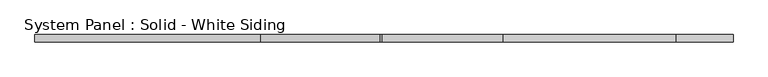
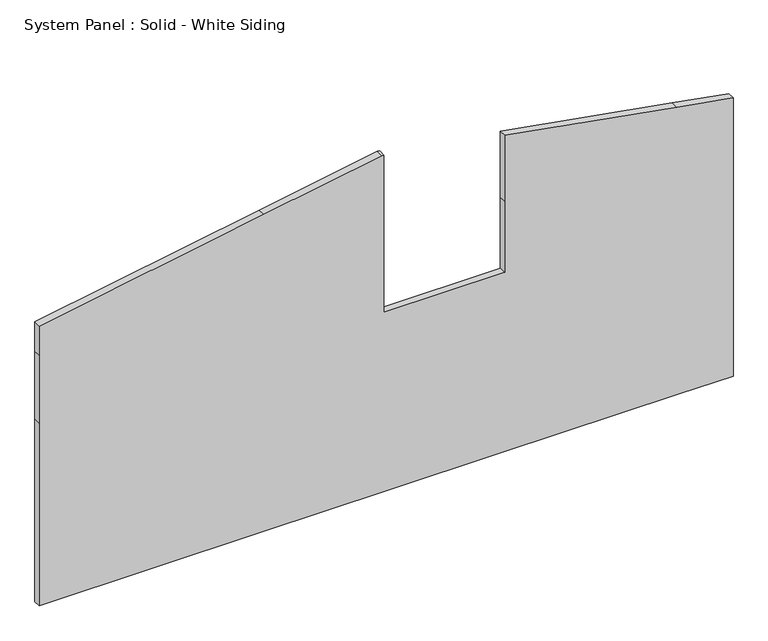
"""IFC4 building model written with IfcOpenShell, lengths in millimetres: plate geometry, System Panel : Solid - White Siding."""

import ifcopenshell
import ifcopenshell.guid

model = None  # the IFC model being written
_history = None  # IfcOwnerHistory: only IFC2X3 demands one
_inside = {}  # id of a spatial element -> (the spatial element, [elements in it])
_under = {}  # id of a project, library or spatial element -> (it, [spatial elements below it])
_declared = {}  # id of a project -> (the project, [libraries it declares])
_typed = {}  # id of a type object -> (the type object, [elements of that type])
_made_of = {}  # id of a material, layer set ... -> (it, [elements and type objects made of it])


def new_model(schema):
    """Start an empty IFC model of exactly this schema.

    Asked for "IFC4X3", IfcOpenShell would pick the latest addendum, in which some entities
    have other attributes; the version numbers below select the first issue.
    IFC2X3 requires an IfcOwnerHistory on every rooted entity: one is made here for all.
    """
    global model, _history
    if schema == "IFC4X3":
        model = ifcopenshell.file(schema_version=(4, 3, 0, 0))
    else:
        model = ifcopenshell.file(schema=schema)
    _inside.clear()
    _under.clear()
    _declared.clear()
    _typed.clear()
    _made_of.clear()
    _history = None
    if model.schema == "IFC2X3":
        org = make("IfcOrganization", Name="unknown")
        user = make(
            "IfcPersonAndOrganization",
            ThePerson=make("IfcPerson", FamilyName="unknown"),
            TheOrganization=org,
        )
        app = make(
            "IfcApplication",
            ApplicationDeveloper=org,
            Version="unknown",
            ApplicationFullName="unknown",
            ApplicationIdentifier="unknown",
        )
        _history = make(
            "IfcOwnerHistory",
            OwningUser=user,
            OwningApplication=app,
            ChangeAction="ADDED",
            CreationDate=0,
        )
    return model


def make(cls, **values):
    """One entity of the class cls with the attributes given. An attribute that is None is left unset."""
    return model.create_entity(
        cls, **{name: value for name, value in values.items() if value is not None}
    )


def rooted(cls, **values):
    """An entity with a GlobalId (a new one), such as an element, a storey or a relation."""
    return make(cls, GlobalId=ifcopenshell.guid.new(), OwnerHistory=_history, **values)


def si_unit(unit_type, name, prefix=None):
    """IfcSIUnit, for example si_unit("LENGTHUNIT", "METRE", prefix="MILLI")."""
    return make("IfcSIUnit", UnitType=unit_type, Prefix=prefix, Name=name)


def assignment(units):
    """IfcUnitAssignment: the units of a project."""
    return None if units is None else make("IfcUnitAssignment", Units=units)


def point(xyz):
    """IfcCartesianPoint."""
    return None if xyz is None else make("IfcCartesianPoint", Coordinates=xyz)


def direction(xyz):
    """IfcDirection."""
    return None if xyz is None else make("IfcDirection", DirectionRatios=xyz)


def frame(location, z_axis=None, x_axis=None):
    """IfcAxis2Placement3D, a coordinate frame: its origin and axes. An axis left out is left unset."""
    return make(
        "IfcAxis2Placement3D",
        Location=point(location),
        Axis=direction(z_axis),
        RefDirection=direction(x_axis),
    )


def origin():
    """The frame at (0, 0, 0) with its axes left unset."""
    return frame((0.0, 0.0, 0.0))


def place(relative_to, where):
    """IfcLocalPlacement: puts the frame where relative to a parent placement (None: the world)."""
    return make(
        "IfcLocalPlacement", PlacementRelTo=relative_to, RelativePlacement=where
    )


def context(
    kind, dimensions, precision=None, world=None, true_north=None, identifier=None
):
    """IfcGeometricRepresentationContext, for example the 3D "Model" context."""
    return make(
        "IfcGeometricRepresentationContext",
        ContextIdentifier=identifier,
        ContextType=kind,
        CoordinateSpaceDimension=dimensions,
        Precision=precision,
        WorldCoordinateSystem=world,
        TrueNorth=true_north,
    )


def project(units=None, contexts=None):
    """IfcProject with its units and contexts."""
    return rooted(
        "IfcProject",
        Name="project",
        RepresentationContexts=contexts,
        UnitsInContext=assignment(units),
    )


def spatial(cls, under=None, at=None, **own):
    """A site, building, storey or space (cls), placed at a placement, below another one or the project."""
    s = rooted(cls, ObjectPlacement=at, **own)
    if under is not None:
        _under.setdefault(under.id(), (under, []))[1].append(s)
    return s


def polyline(points):
    """IfcPolyline through the points."""
    return make("IfcPolyline", Points=[point(p) for p in points])


def outline(outer, holes=None, kind="AREA"):
    """IfcArbitraryClosedProfileDef: a profile drawn as a closed curve; with holes, ...WithVoids."""
    if holes is None:
        return make("IfcArbitraryClosedProfileDef", ProfileType=kind, OuterCurve=outer)
    return make(
        "IfcArbitraryProfileDefWithVoids",
        ProfileType=kind,
        OuterCurve=outer,
        InnerCurves=holes,
    )


def extrude(swept, where, along, depth):
    """IfcExtrudedAreaSolid: the profile swept, set in the frame where, extruded along a direction by depth."""
    return make(
        "IfcExtrudedAreaSolid",
        SweptArea=swept,
        Position=where,
        ExtrudedDirection=direction(along),
        Depth=depth,
    )


def shape(context_of_items, identifier, shape_type, items):
    """IfcShapeRepresentation: the items that make up one representation, for example the "Body"."""
    return make(
        "IfcShapeRepresentation",
        ContextOfItems=context_of_items,
        RepresentationIdentifier=identifier,
        RepresentationType=shape_type,
        Items=items,
    )


def source(mapping_origin, context_of_items, identifier, shape_type, items):
    """IfcRepresentationMap: a shape defined once, which mapped items show again and again."""
    return make(
        "IfcRepresentationMap",
        MappingOrigin=mapping_origin,
        MappedRepresentation=shape(context_of_items, identifier, shape_type, items),
    )


def transform(
    local_origin,
    x_axis=None,
    y_axis=None,
    z_axis=None,
    scale=None,
    scale2=None,
    scale3=None,
    uniform=True,
):
    """IfcCartesianTransformationOperator3D, or its non-uniform kind. x_axis, y_axis, z_axis: its Axis1, 2, 3."""
    if uniform:
        return make(
            "IfcCartesianTransformationOperator3D",
            Axis1=direction(x_axis),
            Axis2=direction(y_axis),
            LocalOrigin=point(local_origin),
            Scale=scale,
            Axis3=direction(z_axis),
        )
    return make(
        "IfcCartesianTransformationOperator3DnonUniform",
        Axis1=direction(x_axis),
        Axis2=direction(y_axis),
        LocalOrigin=point(local_origin),
        Scale=scale,
        Axis3=direction(z_axis),
        Scale2=scale2,
        Scale3=scale3,
    )


def mapped(mapping_source, mapping_target):
    """IfcMappedItem: shows the shape of a source again, moved by a transform."""
    return make(
        "IfcMappedItem", MappingSource=mapping_source, MappingTarget=mapping_target
    )


def made_of(thing, what):
    """Note that an element or type object is made of a material, layer set ...; save() writes the relation."""
    if what is not None:
        _made_of.setdefault(what.id(), (what, []))[1].append(thing)
    return thing


def element(
    cls,
    number,
    at=None,
    inside=None,
    cuts=None,
    type_object=None,
    material=None,
    context=None,
    identifier="Body",
    shape_type=None,
    held_by="IfcProductDefinitionShape",
    body=None,
    shapes=None,
    **own,
):
    """One element of the class cls, such as IfcWall. Its Tag is "e" and its number.

    at: its placement. inside: the storey or other place that contains it. cuts: it is an
    opening in that element (IfcRelVoidsElement). A single representation is given by context,
    identifier, shape_type and body (its items); several are given by shapes. held_by: the class
    of the entity that holds the representations. save() writes the other relations.
    """
    e = rooted(cls, Tag="e%d" % number, ObjectPlacement=at, **own)
    if body is not None:
        shapes = [shape(context, identifier, shape_type, body)]
    if shapes is not None:
        e.Representation = make(held_by, Representations=shapes)
    if inside is not None:
        _inside.setdefault(inside.id(), (inside, []))[1].append(e)
    if cuts is not None:
        rooted(
            "IfcRelVoidsElement", RelatingBuildingElement=cuts, RelatedOpeningElement=e
        )
    if type_object is not None:
        _typed.setdefault(type_object.id(), (type_object, []))[1].append(e)
    return made_of(e, material)


def aggregate(whole, parts):
    """IfcRelAggregates: a whole, such as a stair, and the parts it consists of."""
    return rooted("IfcRelAggregates", RelatingObject=whole, RelatedObjects=parts)


def save(model, path):
    """Write the relations noted so far, then the file.

    IfcRelAggregates (storeys below a building ...), IfcRelContainedInSpatialStructure (elements
    in a storey), IfcRelDefinesByType, IfcRelAssociatesMaterial and IfcRelDeclares: one each for
    every whole, place, type object, material and project.
    """
    for whole, parts in _under.values():
        aggregate(whole, parts)
    for where, things in _inside.values():
        rooted(
            "IfcRelContainedInSpatialStructure",
            RelatedElements=things,
            RelatingStructure=where,
        )
    for kind, things in _typed.values():
        rooted("IfcRelDefinesByType", RelatedObjects=things, RelatingType=kind)
    for what, things in _made_of.values():
        rooted("IfcRelAssociatesMaterial", RelatedObjects=things, RelatingMaterial=what)
    for by, libraries in _declared.values():
        rooted("IfcRelDeclares", RelatingContext=by, RelatedDefinitions=libraries)
    model.write(path)


def system_panel_solid_white_siding_d1a1bcec(model_context):
    return source(origin(), model_context, "Body", "SweptSolid", [
        extrude(outline(polyline([(0.0, -2959.1), (0.0, -1055.3257062), (0.0, 12.7), (0.0, 979.1257062), (0.0, 2489.2), (0.0, 2959.1), (1647.8580051, 2959.1), (2257.4580051, 2959.1), (2508.9751785, 2959.1), (2593.7755243, 2478.1733407), (2852.499686, 1010.8757062), (2257.4580051, 1010.8757062), (1616.1080051, 1010.8757062), (1616.1080051, -19.05), (2257.4580051, -19.05), (3034.1033761, -19.05), (3037.4624051, -38.1), (2860.0423651, -1044.2990469), (2522.4112944, -2959.1), (2257.4580051, -2959.1), (1647.8580051, -2959.1), (0.0, -2959.1)])), frame((0.0, -44.45, 0.0), z_axis=(0.0, 1.0, 0.0), x_axis=(0.0, 0.0, 1.0)), (0.0, 0.0, 1.0), 63.5),
    ])


if __name__ == "__main__":
    model = new_model("IFC4")
    model_context = context("Model", 3, world=origin())
    ifc_project = project(units=[si_unit("LENGTHUNIT", "METRE", prefix="MILLI")], contexts=[model_context])
    site = spatial("IfcSite", under=ifc_project)
    building = spatial("IfcBuilding", under=site)
    placement = place(None, origin())
    system_panel_solid_white_siding_shape = system_panel_solid_white_siding_d1a1bcec(model_context)
    element("IfcPlate", 1, ObjectType="System Panel : Solid - White Siding", at=placement, inside=building, context=model_context, shape_type="MappedRepresentation", body=[
        mapped(system_panel_solid_white_siding_shape, transform((0.0, 0.0, 0.0), x_axis=(1.0, 0.0, 0.0), y_axis=(0.0, 1.0, 0.0), z_axis=(0.0, 0.0, 1.0))),
    ])
    save(model, "model.ifc")

# Revit data of these elements
# Element 1 (IfcPlate, "System Panel : Solid - White Siding")
#   Materials on its faces: "White Siding"
# Materials
#   "White Siding": class "Unassigned", colour RGB 255 255 255, transparency 0
